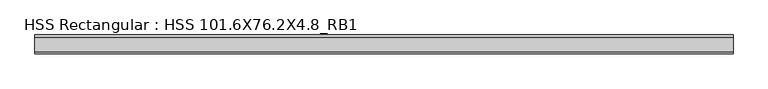
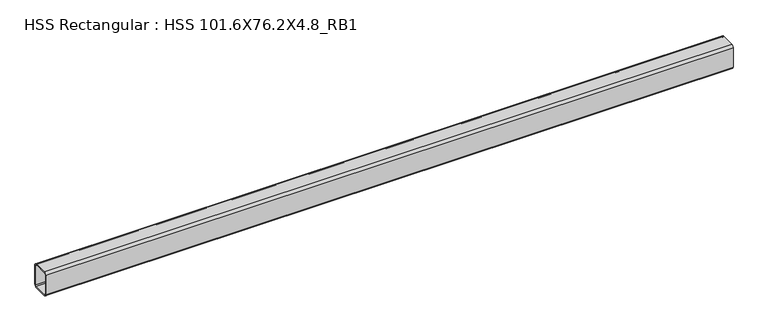
"""IFC4 building model written with IfcOpenShell, lengths in millimetres: beam geometry, HSS Rectangular : HSS 101.6X76.2X4.8_RB1."""

from ifc_helpers import new_model, si_unit, point, frame, frame_2d, origin, place, context, project, spatial, polyline, circle_curve, trimmed, segment, composite_curve, outline, extrude, source, transform, mapped, element, save


def hss_rectangular_hss_101_6x76_2x4_8_rb1_c969aa20(model_context):
    return source(origin(), model_context, "Body", "SweptSolid", [
        extrude(outline(composite_curve([segment(polyline([(38.1, 41.275), (38.1, -41.275)]), True, "CONTINUOUS"), segment(trimmed(circle_curve(frame_2d((28.575, -41.275)), 9.525), [point((38.1, -41.275))], [point((28.575, -50.8))], False, "CARTESIAN"), True, "CONTINUOUS"), segment(polyline([(28.575, -50.8), (-28.575, -50.8)]), True, "CONTINUOUS"), segment(trimmed(circle_curve(frame_2d((-28.575, -41.275)), 9.525), [point((-28.575, -50.8))], [point((-38.1, -41.275))], False, "CARTESIAN"), True, "CONTINUOUS"), segment(polyline([(-38.1, -41.275), (-38.1, 41.275)]), True, "CONTINUOUS"), segment(trimmed(circle_curve(frame_2d((-28.575, 41.275)), 9.525), [point((-38.1, 41.275))], [point((-28.575, 50.8))], False, "CARTESIAN"), True, "CONTINUOUS"), segment(polyline([(-28.575, 50.8), (28.575, 50.8)]), True, "CONTINUOUS"), segment(trimmed(circle_curve(frame_2d((28.575, 41.275)), 9.525), [point((28.575, 50.8))], [point((38.1, 41.275))], False, "CARTESIAN"), True, "CONTINUOUS")], self_intersect=False), holes=[composite_curve([segment(trimmed(circle_curve(frame_2d((-28.575, 41.275)), 4.7625), [point((-28.575, 46.0375))], [point((-33.3375, 41.275))], True, "CARTESIAN"), True, "CONTINUOUS"), segment(polyline([(-33.3375, 41.275), (-33.3375, -41.275)]), True, "CONTINUOUS"), segment(trimmed(circle_curve(frame_2d((-28.575, -41.275)), 4.7625), [point((-33.3375, -41.275))], [point((-28.575, -46.0375))], True, "CARTESIAN"), True, "CONTINUOUS"), segment(polyline([(-28.575, -46.0375), (28.575, -46.0375)]), True, "CONTINUOUS"), segment(trimmed(circle_curve(frame_2d((28.575, -41.275)), 4.7625), [point((28.575, -46.0375))], [point((33.3375, -41.275))], True, "CARTESIAN"), True, "CONTINUOUS"), segment(polyline([(33.3375, -41.275), (33.3375, 41.275)]), True, "CONTINUOUS"), segment(trimmed(circle_curve(frame_2d((28.575, 41.275)), 4.7625), [point((33.3375, 41.275))], [point((28.575, 46.0375))], True, "CARTESIAN"), True, "CONTINUOUS"), segment(polyline([(28.575, 46.0375), (-28.575, 46.0375)]), True, "CONTINUOUS")], self_intersect=False)]), frame((-1385.225, 0.0, 0.0), z_axis=(1.0, 0.0, 0.0), x_axis=(0.0, 1.0, 0.0)), (0.0, 0.0, 1.0), 2795.85),
    ])


if __name__ == "__main__":
    model = new_model("IFC4")
    model_context = context("Model", 3, world=origin())
    ifc_project = project(units=[si_unit("LENGTHUNIT", "METRE", prefix="MILLI")], contexts=[model_context])
    site = spatial("IfcSite", under=ifc_project)
    building = spatial("IfcBuilding", under=site)
    placement = place(None, origin())
    hss_rectangular_hss_101_6x76_2x4_8_rb1_shape = hss_rectangular_hss_101_6x76_2x4_8_rb1_c969aa20(model_context)
    element("IfcBeam", 1, ObjectType="HSS Rectangular : HSS 101.6X76.2X4.8_RB1", at=placement, inside=building, context=model_context, shape_type="MappedRepresentation", body=[
        mapped(hss_rectangular_hss_101_6x76_2x4_8_rb1_shape, transform((0.0, 0.0, 0.0), x_axis=(1.0, 0.0, 0.0), y_axis=(0.0, 1.0, 0.0), z_axis=(0.0, 0.0, 1.0))),
    ])
    save(model, "model.ifc")

# Revit data of these elements
# Type "HSS Rectangular : HSS 101.6X76.2X4.8_RB1"
#   Section Name Key = "HSS 4X3X3/16"
#   Assembly Code = "B10"
#   Width = 7.62 cm
#   Wall Nominal Thickness = 0.4763 cm
#   Wall Design Thickness = 0.442 cm
#   Torsional Moment of Inertia = 260.561 cm⁴
#   Torsional Modulus = 61.2876 cm³
#   Section Area = 14.4516 cm²
#   Plastic Modulus weak axis = 40.3122 cm³
#   Plastic Modulus strong axis = 49.1612 cm³
#   Perimeter = 0.881482 m²/m
#   Outer Fillet = 0.9525 cm
#   Nominal Weight = 12.1285 kgf/m
#   Moment of Inertia weak axis = 131.529 cm⁴
#   Moment of Inertia strong axis = 205.202 cm⁴
#   Inner Fillet = 0.4763 cm
#   Height = 10.16 cm
#   Elastic Modulus weak axis = 34.4128 cm³
#   Elastic Modulus strong axis = 40.476 cm³
#   Centroid Vertical = 5.08 cm
#   Centroid Horizontal = 3.81 cm
#   Length [instance default] = 1524 mm
#   Structural Material [instance default] = Steel ASTM A500, Grade B, Rectangular and Square
#   Principal Axes Angle = 0
# Element 1 (IfcBeam, "HSS Rectangular : HSS 101.6X76.2X4.8_RB1")
#   Structural Material = Steel ASTM A992
#   Materials on its faces: "Steel ASTM A992"
# Materials
#   "Steel ASTM A500, Grade B, Rectangular and Square": class "Metal", colour RGB 199 199 199, transparency 0, Description = "Carbon steel", Cost = 0
#   "Steel ASTM A992": class "Metal", colour RGB 199 199 199, transparency 0, Description = "Structural steel 50ksi", Cost = 0
